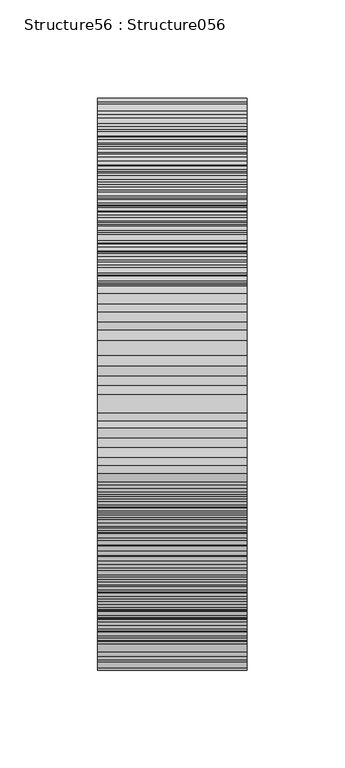
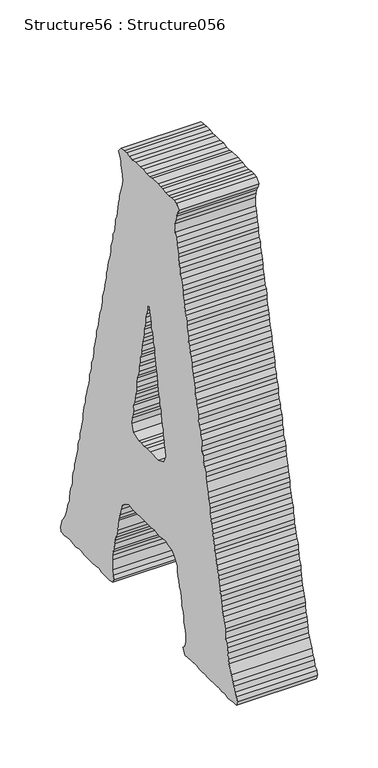
"""IFC4 building model written with IfcOpenShell, lengths in millimetres: proxy geometry, Structure56 : Structure056."""

from ifc_helpers import new_model, si_unit, frame, origin, place, context, project, spatial, polyline, outline, extrude, source, transform, mapped, element, save


def structure56_structure056_6db47774(model_context):
    return source(origin(), model_context, "Body", "SweptSolid", [
        extrude(outline(polyline([(254723.7661623, 3818.8310229), (254726.1072802, 3824.1149855), (254726.6865425, 3828.2163546), (254727.2658047, 3833.4730389), (254729.0260558, 3838.1761347), (254729.6277825, 3841.6741725), (254731.3655692, 3846.9757858), (254731.3655692, 3851.6612309), (254733.1274249, 3856.9179152), (254734.3084138, 3861.0192843), (254735.4669383, 3866.3032469), (254736.6479272, 3870.4030114), (254737.2271894, 3875.0772243), (254738.9874405, 3878.5784713), (254739.5683073, 3884.4609514), (254739.5683073, 3888.5623205), (254740.7492963, 3893.822214), (254742.5095474, 3896.763454), (254743.6905363, 3902.6314927), (254744.8490607, 3906.1487857), (254746.0300496, 3910.8310217), (254746.0300496, 3915.5068392), (254747.1901787, 3919.6066036), (254748.9504298, 3924.8905662), (254750.710681, 3929.5904528), (254750.710681, 3934.8503464), (254752.4709321, 3938.3499888), (254753.6294565, 3944.235678), (254753.6294565, 3947.7337158), (254755.3913123, 3952.435207), (254755.993039, 3957.1190475), (254757.1515634, 3962.3757319), (254758.9118145, 3966.5043792), (254758.9118145, 3974.7055128), (254757.7308256, 3979.3781211), (254756.5723012, 3984.0635662), (254754.8120501, 3987.5792547), (254752.4709321, 3992.2614906), (254756.5723012, 3996.9645864), (254760.6720657, 3997.5486624), (254764.7734348, 3997.5486624), (254770.0557928, 3996.390138), (254774.7348195, 3996.390138), (254779.994713, 3997.5486624), (254783.5152153, 3996.9645864), (254787.6165844, 3997.5486624), (254796.9987068, 3997.5486624), (254801.6793382, 3996.390138), (254806.3808293, 3996.390138), (254811.6407229, 3997.5486624), (254816.9230809, 3996.9645864), (254824.5224878, 3996.9645864), (254829.8048458, 3996.390138), (254833.9046102, 3997.5486624), (254839.1869682, 3997.5486624), (254843.2867327, 3996.9645864), (254848.5690907, 3996.390138), (254852.0687331, 3991.6806238), (254849.7276152, 3987.5792547), (254848.5690907, 3983.4794902), (254847.967364, 3979.9621971), (254846.8088396, 3974.7055128), (254845.0485885, 3965.8930249), (254846.2071129, 3961.794865), (254847.3881018, 3956.5349715), (254850.9086041, 3947.1496398), (254850.9086041, 3944.235678), (254852.0687331, 3938.9517154), (254853.249722, 3934.2758979), (254853.8289843, 3928.9919353), (254855.0099732, 3924.2888396), (254857.3494865, 3919.6066036), (254857.3494865, 3916.0909152), (254857.9287488, 3910.8310217), (254859.1113423, 3906.1487857), (254861.4508556, 3902.6314927), (254861.4508556, 3897.3475301), (254863.2111068, 3892.6636896), (254864.3920957, 3888.5623205), (254864.3920957, 3883.8881076), (254865.5506201, 3878.5784713), (254867.3124758, 3873.9203044), (254869.072727, 3869.8189354), (254869.6519892, 3866.3032469), (254870.2312514, 3861.0192843), (254871.9915026, 3856.9179152), (254871.9915026, 3851.6612309), (254873.7533583, 3846.9757858), (254874.3326205, 3842.8583706), (254875.5136094, 3837.6000817), (254878.432385, 3829.374879), (254878.432385, 3824.1149855), (254879.6133739, 3820.015221), (254880.773503, 3815.3313805), (254883.1354808, 3810.0474179), (254883.714743, 3806.5317294), (254884.8732675, 3801.8462843), (254885.4749941, 3797.1463977), (254887.2352453, 3791.8865042), (254888.3953743, 3788.3611881), (254888.3953743, 3783.0868532), (254890.1556254, 3777.8285642), (254890.7573521, 3774.3032481), (254892.4951388, 3769.0176809), (254893.0968655, 3764.3611187), (254893.6761277, 3759.6596275), (254894.8571166, 3756.1423345), (254896.5965079, 3751.4424479), (254897.1982346, 3745.6000829), (254898.356759, 3740.9162424), (254900.1170102, 3737.9750024), (254900.1170102, 3732.7167134), (254901.2979991, 3727.4311462), (254903.0373903, 3723.3313817), (254904.2183792, 3718.0554422), (254905.3993682, 3714.5301261), (254906.5578926, 3710.4560353), (254906.5578926, 3705.7545441), (254908.9198704, 3699.8881101), (254910.0783949, 3695.2122926), (254910.6592617, 3691.0868544), (254910.6592617, 3686.4030139), (254911.8402506, 3682.8857208), (254913.6005017, 3677.0449604), (254914.179764, 3673.5276674), (254915.9400151, 3668.8261762), (254915.9400151, 3663.5598643), (254918.281133, 3659.4584952), (254919.462122, 3655.3587307), (254919.462122, 3650.6845178), (254920.6431109, 3645.4262289), (254922.3808975, 3640.114988), (254923.5618864, 3636.0408972), (254924.7428754, 3632.5155811), (254925.3012777, 3627.2396415), (254927.0839933, 3622.555801), (254928.2425178, 3617.2718384), (254928.2425178, 3612.5976255), (254928.82178, 3608.4705827), (254931.1837578, 3604.3964919), (254932.3422822, 3599.1125293), (254933.5248758, 3594.4286888), (254933.5248758, 3590.3289243), (254935.2851269, 3586.2115092), (254938.2039025, 3576.2693797), (254939.9641536, 3572.1423369), (254941.7260093, 3568.6426945), (254945.2465116, 3563.366755), (254946.405036, 3560.441561), (254948.1668918, 3555.1848766), (254947.0067627, 3551.0658569), (254941.1242827, 3550.4833855), (254937.6246402, 3551.0658569), (254932.3422822, 3551.6675836), (254927.6632555, 3550.4833855), (254922.3808975, 3550.4833855), (254917.7002662, 3551.6675836), (254913.6005017, 3551.6675836), (254908.9198704, 3551.0658569), (254904.8201059, 3551.0658569), (254898.9360213, 3550.4833855), (254894.8571166, 3550.4833855), (254890.1556254, 3551.0658569), (254884.8732675, 3551.6675836), (254880.773503, 3550.4833855), (254867.3124758, 3550.4833855), (254862.0301178, 3551.6675836), (254859.6906045, 3555.7416744), (254861.4508556, 3559.2669905), (254862.6093801, 3563.9412034), (254862.6093801, 3573.9266571), (254862.6093801, 3578.6104977), (254861.4508556, 3582.7102621), (254859.6906045, 3586.2115092), (254859.1113423, 3592.0955938), (254857.9287488, 3596.1953583), (254856.1684976, 3600.2967274), (254855.0099732, 3604.3964919), (254853.8289843, 3609.0723094), (254852.6704598, 3619.6145609), (254851.4894709, 3622.555801), (254849.7276152, 3627.2396415), (254848.5690907, 3633.0980525), (254845.6278507, 3638.9580681), (254841.5264816, 3642.4833842), (254835.0855992, 3645.9830266), (254830.4065724, 3644.8245022), (254821.0228454, 3644.8245022), (254815.1628297, 3645.4262289), (254802.8603271, 3645.4262289), (254797.5779691, 3644.8245022), (254793.4782046, 3645.9830266), (254788.7975733, 3645.4262289), (254784.116942, 3644.8245022), (254779.994713, 3645.4262289), (254774.1555572, 3645.9830266), (254770.635055, 3644.8245022), (254763.6149103, 3643.0578326), (254760.070339, 3639.5405396), (254755.3913123, 3633.0980525), (254755.3913123, 3627.8397636), (254754.2311832, 3622.555801), (254752.4709321, 3619.6145609), (254751.8916699, 3613.772196), (254749.5296921, 3610.2292293), (254748.3711676, 3604.9709403), (254747.7919054, 3601.4536473), (254747.7919054, 3596.7698067), (254745.428323, 3592.0955938), (254744.8490607, 3587.3860796), (254744.2697985, 3582.7102621), (254742.5095474, 3578.6104977), (254740.7492963, 3572.7440636), (254741.3285585, 3565.1254015), (254743.0888096, 3559.2669905), (254746.0300496, 3556.3417965), (254742.5095474, 3550.4833855), (254737.2271894, 3551.0658569), (254732.5481627, 3551.6675836), (254723.1644356, 3551.6675836), (254718.4854089, 3551.0658569), (254713.8047776, 3551.0658569), (254709.7034085, 3551.6675836), (254705.603644, 3551.0658569), (254699.7420238, 3551.0658569), (254696.2215215, 3551.6675836), (254690.3599013, 3551.0658569), (254686.8377944, 3551.6675836), (254682.1587677, 3550.4833855), (254676.8764097, 3551.6675836), (254671.6165162, 3550.4833855), (254667.5167517, 3551.0658569), (254662.8136559, 3551.6675836), (254658.1346292, 3551.6675836), (254656.3727735, 3556.3417965), (254657.5537624, 3560.441561), (254660.4741425, 3563.366755), (254661.6551315, 3568.6426945), (254663.4153826, 3572.1423369), (254665.7565005, 3577.4535778), (254669.856265, 3586.2115092), (254671.0147895, 3589.7544759), (254671.6165162, 3595.5872132), (254672.7766452, 3600.2967274), (254673.9576341, 3604.3964919), (254675.7178853, 3607.8961343), (254676.2971475, 3613.772196), (254676.2971475, 3617.2718384), (254677.4781364, 3622.555801), (254679.2159231, 3627.8397636), (254681.0002433, 3631.915459), (254682.1587677, 3636.0408972), (254682.7380299, 3641.2991861), (254683.3397566, 3645.9830266), (254683.9190188, 3650.1004418), (254686.2585322, 3654.1841602), (254686.8377944, 3660.0682449), (254687.4395211, 3664.1423357), (254688.0203879, 3668.8261762), (254689.7806391, 3672.9435914), (254691.5408902, 3677.6274319), (254692.6994146, 3682.8857208), (254693.8804035, 3685.8285655), (254693.8804035, 3690.512406), (254695.6422593, 3695.786741), (254696.2215215, 3701.0723082), (254697.3800459, 3704.5879966), (254699.1627615, 3709.2718371), (254699.7420238, 3713.3555556), (254701.4798104, 3718.6571688), (254701.4798104, 3723.3313817), (254702.6624039, 3727.4311462), (254703.8209284, 3732.1149867), (254705.0019173, 3737.400554), (254707.3638951, 3746.1745313), (254708.5224196, 3750.8583719), (254708.5224196, 3755.559863), (254710.2842753, 3759.6596275), (254712.0445264, 3763.759392), (254712.0445264, 3769.6274306), (254714.3840398, 3773.11905), (254714.3840398, 3777.8285642), (254714.963302, 3783.0868532), (254717.30442, 3787.7867397), (254717.30442, 3791.8865042), (254719.6439333, 3795.960595), (254720.24566, 3801.8462843), (254720.24566, 3805.9476534), (254722.5851734, 3811.2043377), (254723.7661623, 3814.7296538), (254723.7661623, 3818.8310229)]), holes=[polyline([(254786.4580599, 3720.4158154), (254799.919087, 3720.4158154), (254805.1998404, 3720.9726131), (254810.4821984, 3719.8140887), (254814.5835675, 3720.9726131), (254818.683332, 3720.4158154), (254827.4637278, 3723.3313817), (254830.4065724, 3730.9323932), (254829.2255835, 3736.7988273), (254828.04299, 3740.9162424), (254826.8844656, 3744.9999608), (254827.4637278, 3750.8583719), (254825.1242144, 3754.9854146), (254824.5224878, 3759.6596275), (254823.9432255, 3763.759392), (254822.2054389, 3767.8607611), (254821.6037122, 3772.5606477), (254821.6037122, 3777.2444882), (254821.0228454, 3782.5027771), (254819.2625942, 3786.0280932), (254818.0816053, 3790.7039107), (254818.0816053, 3795.4037973), (254815.742092, 3800.6717138), (254815.742092, 3805.9476534), (254813.9818408, 3810.0474179), (254813.400974, 3813.5743386), (254812.8217118, 3819.4150989), (254811.6407229, 3824.1149855), (254810.4821984, 3828.790803), (254809.8804717, 3832.8921721), (254809.8804717, 3837.6000817), (254807.5409584, 3842.2758992), (254806.9616962, 3846.3772683), (254806.9616962, 3851.6612309), (254805.1998404, 3856.3161885), (254804.041316, 3860.4432313), (254804.041316, 3864.5446004), (254802.2586004, 3865.1190488), (254801.1000759, 3860.4432313), (254799.3398248, 3855.7353217), (254798.758958, 3851.0595042), (254798.758958, 3845.8012153), (254796.4194446, 3842.2758992), (254795.8177179, 3836.9919366), (254795.8177179, 3833.4730389), (254793.4782046, 3828.790803), (254792.8989424, 3822.932392), (254792.3196801, 3818.8310229), (254791.1370866, 3814.7296538), (254790.5578244, 3810.0474179), (254788.7975733, 3804.7730829), (254788.218311, 3795.4037973), (254787.0373221, 3790.7039107), (254786.4580599, 3786.0280932), (254784.6978088, 3783.0868532), (254784.6978088, 3777.8285642), (254782.3566908, 3773.11905), (254782.3566908, 3768.4432325), (254781.1757019, 3764.3611187), (254780.5964397, 3759.0595054), (254778.8361886, 3755.559863), (254778.8361886, 3750.3015741), (254777.0759374, 3744.9999608), (254777.0759374, 3741.5003184), (254775.8933439, 3736.7988273), (254774.7348195, 3730.9323932), (254778.2569263, 3723.9154578), (254786.4580599, 3720.4158154)])]), frame((-38594.2176606, 0.0, 0.0), z_axis=(1.0, 0.0, 0.0), x_axis=(0.0, 1.0, 0.0)), (0.0, 0.0, 1.0), 76.2),
    ])


if __name__ == "__main__":
    model = new_model("IFC4")
    model_context = context("Model", 3, world=origin())
    ifc_project = project(units=[si_unit("LENGTHUNIT", "METRE", prefix="MILLI")], contexts=[model_context])
    site = spatial("IfcSite", under=ifc_project)
    building = spatial("IfcBuilding", under=site)
    placement = place(None, origin())
    structure56_structure056_shape = structure56_structure056_6db47774(model_context)
    element("IfcBuildingElementProxy", 1, Name="Structure56 : Structure056", ObjectType="Structure56 : Structure056", at=placement, inside=building, context=model_context, shape_type="MappedRepresentation", body=[
        mapped(structure56_structure056_shape, transform((0.0, 0.0, 0.0), x_axis=(1.0, 0.0, 0.0), y_axis=(0.0, 1.0, 0.0), z_axis=(0.0, 0.0, 1.0))),
    ])
    save(model, "model.ifc")

# Revit data of these elements
# Type "Structure56 : Structure056"
#   NameOverride = "Structure056"
# Element 1 (IfcBuildingElementProxy, "Structure56 : Structure056")
#   Materials on its faces: "BRUSHED ALUM. LETTERING"
# Materials
#   "BRUSHED ALUM. LETTERING": class "Unassigned", colour RGB 169 181 186, transparency 0, Cost = 0
